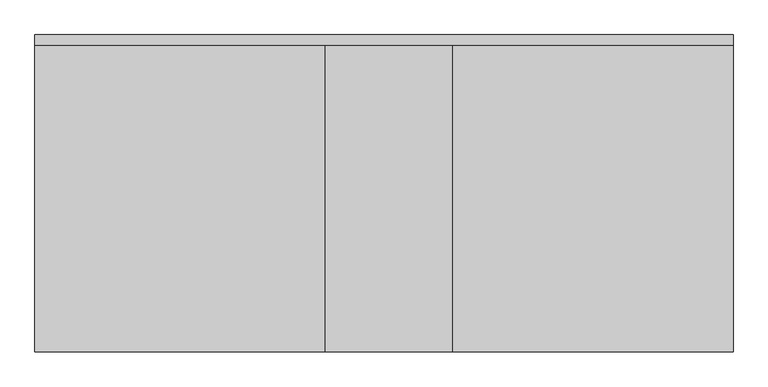
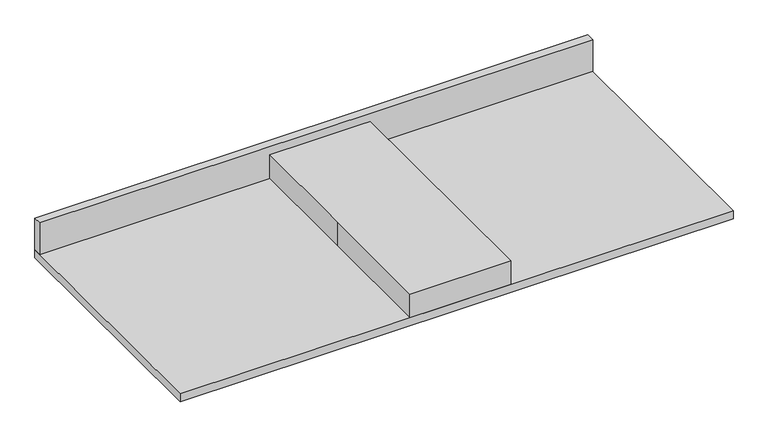
"""IFC4 building model written with IfcOpenShell, lengths in millimetres: proxy geometry, CT050 - Countertop, Stainless Steel (w-o opening) : CT050 - Countertop, Stainless Steel (w-o opening)."""

import ifcopenshell
import ifcopenshell.guid

model = None  # the IFC model being written
_history = None  # IfcOwnerHistory: only IFC2X3 demands one
_inside = {}  # id of a spatial element -> (the spatial element, [elements in it])
_under = {}  # id of a project, library or spatial element -> (it, [spatial elements below it])
_declared = {}  # id of a project -> (the project, [libraries it declares])
_typed = {}  # id of a type object -> (the type object, [elements of that type])
_made_of = {}  # id of a material, layer set ... -> (it, [elements and type objects made of it])


def new_model(schema):
    """Start an empty IFC model of exactly this schema.

    Asked for "IFC4X3", IfcOpenShell would pick the latest addendum, in which some entities
    have other attributes; the version numbers below select the first issue.
    IFC2X3 requires an IfcOwnerHistory on every rooted entity: one is made here for all.
    """
    global model, _history
    if schema == "IFC4X3":
        model = ifcopenshell.file(schema_version=(4, 3, 0, 0))
    else:
        model = ifcopenshell.file(schema=schema)
    _inside.clear()
    _under.clear()
    _declared.clear()
    _typed.clear()
    _made_of.clear()
    _history = None
    if model.schema == "IFC2X3":
        org = make("IfcOrganization", Name="unknown")
        user = make(
            "IfcPersonAndOrganization",
            ThePerson=make("IfcPerson", FamilyName="unknown"),
            TheOrganization=org,
        )
        app = make(
            "IfcApplication",
            ApplicationDeveloper=org,
            Version="unknown",
            ApplicationFullName="unknown",
            ApplicationIdentifier="unknown",
        )
        _history = make(
            "IfcOwnerHistory",
            OwningUser=user,
            OwningApplication=app,
            ChangeAction="ADDED",
            CreationDate=0,
        )
    return model


def make(cls, **values):
    """One entity of the class cls with the attributes given. An attribute that is None is left unset."""
    return model.create_entity(
        cls, **{name: value for name, value in values.items() if value is not None}
    )


def rooted(cls, **values):
    """An entity with a GlobalId (a new one), such as an element, a storey or a relation."""
    return make(cls, GlobalId=ifcopenshell.guid.new(), OwnerHistory=_history, **values)


def si_unit(unit_type, name, prefix=None):
    """IfcSIUnit, for example si_unit("LENGTHUNIT", "METRE", prefix="MILLI")."""
    return make("IfcSIUnit", UnitType=unit_type, Prefix=prefix, Name=name)


def assignment(units):
    """IfcUnitAssignment: the units of a project."""
    return None if units is None else make("IfcUnitAssignment", Units=units)


def point(xyz):
    """IfcCartesianPoint."""
    return None if xyz is None else make("IfcCartesianPoint", Coordinates=xyz)


def direction(xyz):
    """IfcDirection."""
    return None if xyz is None else make("IfcDirection", DirectionRatios=xyz)


def frame(location, z_axis=None, x_axis=None):
    """IfcAxis2Placement3D, a coordinate frame: its origin and axes. An axis left out is left unset."""
    return make(
        "IfcAxis2Placement3D",
        Location=point(location),
        Axis=direction(z_axis),
        RefDirection=direction(x_axis),
    )


def origin():
    """The frame at (0, 0, 0) with its axes left unset."""
    return frame((0.0, 0.0, 0.0))


def origin_with_axes():
    """The frame at (0, 0, 0) with the z axis (0, 0, 1) and the x axis (1, 0, 0) written out."""
    return frame((0.0, 0.0, 0.0), z_axis=(0.0, 0.0, 1.0), x_axis=(1.0, 0.0, 0.0))


def place(relative_to, where):
    """IfcLocalPlacement: puts the frame where relative to a parent placement (None: the world)."""
    return make(
        "IfcLocalPlacement", PlacementRelTo=relative_to, RelativePlacement=where
    )


def context(
    kind, dimensions, precision=None, world=None, true_north=None, identifier=None
):
    """IfcGeometricRepresentationContext, for example the 3D "Model" context."""
    return make(
        "IfcGeometricRepresentationContext",
        ContextIdentifier=identifier,
        ContextType=kind,
        CoordinateSpaceDimension=dimensions,
        Precision=precision,
        WorldCoordinateSystem=world,
        TrueNorth=true_north,
    )


def project(units=None, contexts=None):
    """IfcProject with its units and contexts."""
    return rooted(
        "IfcProject",
        Name="project",
        RepresentationContexts=contexts,
        UnitsInContext=assignment(units),
    )


def spatial(cls, under=None, at=None, **own):
    """A site, building, storey or space (cls), placed at a placement, below another one or the project."""
    s = rooted(cls, ObjectPlacement=at, **own)
    if under is not None:
        _under.setdefault(under.id(), (under, []))[1].append(s)
    return s


def polyline(points):
    """IfcPolyline through the points."""
    return make("IfcPolyline", Points=[point(p) for p in points])


def outline(outer, holes=None, kind="AREA"):
    """IfcArbitraryClosedProfileDef: a profile drawn as a closed curve; with holes, ...WithVoids."""
    if holes is None:
        return make("IfcArbitraryClosedProfileDef", ProfileType=kind, OuterCurve=outer)
    return make(
        "IfcArbitraryProfileDefWithVoids",
        ProfileType=kind,
        OuterCurve=outer,
        InnerCurves=holes,
    )


def extrude(swept, where, along, depth):
    """IfcExtrudedAreaSolid: the profile swept, set in the frame where, extruded along a direction by depth."""
    return make(
        "IfcExtrudedAreaSolid",
        SweptArea=swept,
        Position=where,
        ExtrudedDirection=direction(along),
        Depth=depth,
    )


def shape(context_of_items, identifier, shape_type, items):
    """IfcShapeRepresentation: the items that make up one representation, for example the "Body"."""
    return make(
        "IfcShapeRepresentation",
        ContextOfItems=context_of_items,
        RepresentationIdentifier=identifier,
        RepresentationType=shape_type,
        Items=items,
    )


def source(mapping_origin, context_of_items, identifier, shape_type, items):
    """IfcRepresentationMap: a shape defined once, which mapped items show again and again."""
    return make(
        "IfcRepresentationMap",
        MappingOrigin=mapping_origin,
        MappedRepresentation=shape(context_of_items, identifier, shape_type, items),
    )


def transform(
    local_origin,
    x_axis=None,
    y_axis=None,
    z_axis=None,
    scale=None,
    scale2=None,
    scale3=None,
    uniform=True,
):
    """IfcCartesianTransformationOperator3D, or its non-uniform kind. x_axis, y_axis, z_axis: its Axis1, 2, 3."""
    if uniform:
        return make(
            "IfcCartesianTransformationOperator3D",
            Axis1=direction(x_axis),
            Axis2=direction(y_axis),
            LocalOrigin=point(local_origin),
            Scale=scale,
            Axis3=direction(z_axis),
        )
    return make(
        "IfcCartesianTransformationOperator3DnonUniform",
        Axis1=direction(x_axis),
        Axis2=direction(y_axis),
        LocalOrigin=point(local_origin),
        Scale=scale,
        Axis3=direction(z_axis),
        Scale2=scale2,
        Scale3=scale3,
    )


def mapped(mapping_source, mapping_target):
    """IfcMappedItem: shows the shape of a source again, moved by a transform."""
    return make(
        "IfcMappedItem", MappingSource=mapping_source, MappingTarget=mapping_target
    )


def made_of(thing, what):
    """Note that an element or type object is made of a material, layer set ...; save() writes the relation."""
    if what is not None:
        _made_of.setdefault(what.id(), (what, []))[1].append(thing)
    return thing


def element(
    cls,
    number,
    at=None,
    inside=None,
    cuts=None,
    type_object=None,
    material=None,
    context=None,
    identifier="Body",
    shape_type=None,
    held_by="IfcProductDefinitionShape",
    body=None,
    shapes=None,
    **own,
):
    """One element of the class cls, such as IfcWall. Its Tag is "e" and its number.

    at: its placement. inside: the storey or other place that contains it. cuts: it is an
    opening in that element (IfcRelVoidsElement). A single representation is given by context,
    identifier, shape_type and body (its items); several are given by shapes. held_by: the class
    of the entity that holds the representations. save() writes the other relations.
    """
    e = rooted(cls, Tag="e%d" % number, ObjectPlacement=at, **own)
    if body is not None:
        shapes = [shape(context, identifier, shape_type, body)]
    if shapes is not None:
        e.Representation = make(held_by, Representations=shapes)
    if inside is not None:
        _inside.setdefault(inside.id(), (inside, []))[1].append(e)
    if cuts is not None:
        rooted(
            "IfcRelVoidsElement", RelatingBuildingElement=cuts, RelatedOpeningElement=e
        )
    if type_object is not None:
        _typed.setdefault(type_object.id(), (type_object, []))[1].append(e)
    return made_of(e, material)


def aggregate(whole, parts):
    """IfcRelAggregates: a whole, such as a stair, and the parts it consists of."""
    return rooted("IfcRelAggregates", RelatingObject=whole, RelatedObjects=parts)


def save(model, path):
    """Write the relations noted so far, then the file.

    IfcRelAggregates (storeys below a building ...), IfcRelContainedInSpatialStructure (elements
    in a storey), IfcRelDefinesByType, IfcRelAssociatesMaterial and IfcRelDeclares: one each for
    every whole, place, type object, material and project.
    """
    for whole, parts in _under.values():
        aggregate(whole, parts)
    for where, things in _inside.values():
        rooted(
            "IfcRelContainedInSpatialStructure",
            RelatedElements=things,
            RelatingStructure=where,
        )
    for kind, things in _typed.values():
        rooted("IfcRelDefinesByType", RelatedObjects=things, RelatingType=kind)
    for what, things in _made_of.values():
        rooted("IfcRelAssociatesMaterial", RelatedObjects=things, RelatingMaterial=what)
    for by, libraries in _declared.values():
        rooted("IfcRelDeclares", RelatingContext=by, RelatedDefinitions=libraries)
    model.write(path)


def specialty_equipment_aaaa1240(model_context):
    return source(origin(), model_context, "Body", "SweptSolid", [
        extrude(outline(polyline([(-849.3125, 355.6), (-849.3125, 381.0), (827.0875, 381.0), (827.0875, 355.6), (-849.3125, 355.6)])), frame((0.0, 0.0, 25.4), z_axis=(0.0, 0.0, 1.0), x_axis=(1.0, 0.0, 0.0)), (0.0, 0.0, 1.0), 101.6),
        extrude(outline(polyline([(827.0875, 381.0), (827.0875, -381.0), (-849.3125, -381.0), (-849.3125, 381.0), (827.0875, 381.0)])), origin_with_axes(), (0.0, 0.0, 1.0), 25.4),
        extrude(outline(polyline([(-152.4, 381.0), (152.4, 381.0), (152.4, -381.0), (-152.4, -381.0), (-152.4, 0.0), (-152.4, 381.0)])), origin_with_axes(), (0.0, 0.0, 1.0), 101.6),
    ])


if __name__ == "__main__":
    model = new_model("IFC4")
    model_context = context("Model", 3, world=origin())
    ifc_project = project(units=[si_unit("LENGTHUNIT", "METRE", prefix="MILLI")], contexts=[model_context])
    site = spatial("IfcSite", under=ifc_project)
    building = spatial("IfcBuilding", under=site)
    placement = place(None, origin())
    specialty_equipment_shape = specialty_equipment_aaaa1240(model_context)
    element("IfcBuildingElementProxy", 1, Name="CT050 - Countertop, Stainless Steel (w-o opening) : CT050 - Countertop, Stainless Steel (w-o opening)", ObjectType="CT050 - Countertop, Stainless Steel (w-o opening) : CT050 - Countertop, Stainless Steel (w-o opening)", at=placement, inside=building, context=model_context, shape_type="MappedRepresentation", body=[
        mapped(specialty_equipment_shape, transform((0.0, 0.0, 0.0), x_axis=(1.0, 0.0, 0.0), y_axis=(0.0, 1.0, 0.0), z_axis=(0.0, 0.0, 1.0))),
    ])
    save(model, "model.ifc")

# Revit data of these elements
# Project information
#   Room Abbreviation = "CSDE1"
#   Room Description = "Workroom, Sterile Processing, Decontamination (CSDE1)"
#   Sheets - Total = "7"
#   Project Issue Date = "Issue Date"
#   Project Status = "Project Status"
#   Client Name = "Owner"
#   Project Address = "Enter address here"
#   Project Name = "Project Name"
#   Project Number = "Project Number"
#   Publication Date = "30-Jan-15"
# Type "CT050 - Countertop, Stainless Steel (w-o opening) : CT050 - Countertop, Stainless Steel (w-o opening)"
#   Watts2 = "0"
#   Watts1 = "0"
#   Unit_Issue = "LF"
#   UTIL_6_Misc = "-"
#   UTIL_5_NonMedGas = "-"
#   UTIL_4_MiscGas = "-"
#   UTIL_3_MedGas = "-"
#   UTIL_2_Elec = "-"
#   UTIL_1_WaterDrain = "-"
#   Nomenclature = "Countertop, Stainless Steel"
#   NSN = "6530"
#   Location [instance default] = ""
#   JSN = "CT050"
#   Fund_Source_VA = "-"
#   Fund_Source_Navy = "-"
#   Fund_Source_Army = "-"
#   Fund_Source_AF = "-"
#   ELEC_Volts2 = "0"
#   ELEC_Volts1 = "0"
#   ELEC_Phase2 = "0"
#   ELEC_Phase1 = "0"
#   ELEC_HertzSwitch = "0"
#   ELEC_HertzDependent = "0"
#   ELEC_Hertz = "0"
#   ELEC_Amps2 = "0"
#   ELEC_Amps1 = "0"
#   DetailDescription = "Stainless steel countertop (composition of heavy-gauge Type No. 304 stainless steel) having a smooth satin finish and integral 4\" backsplash/curb. Also referred to as a corrosion-resistant steel work surface or work top. Available in various depths. Used in areas where excellent ease of cleaning, abrasion resistance, bacteria resistance, impact resistance, load capacity and moisture resistance, are of concern. Pricing based upon a 24\" depth."
#   CAT_VA = "A"
#   CAT_Navy = "A"
#   CAT_IHS = "-"
#   CAT_Army = "A"
#   CAT_AF = "A"
#   BTUperhour = "0"
#   Weight_IP = 0
#   OpeningLength [instance default] = 1' - 7"
#   OpeningDepth [instance default] = 1' - 4"
#   DIM_Width_IP = 1' - 0"
#   DIM_Height_IP = 0' - 4"
#   DIM_Depth_IP = 2' - 6"
#   CustomLength2 [instance default] = 1' - 6"
#   CustomLength [instance default] = 1' - 6"
#   Assembly Code = ""
# Element 1 (IfcBuildingElementProxy, "CT050 - Countertop, Stainless Steel (w-o opening) : CT050 - Countertop, Stainless Steel (w-o opening)")
#   Location = "CSDE2"
#   CustomLength2 = 2' - 8 9/16"
#   CustomLength = 2' - 9 7/16"
#   Materials on its faces: "CounterTopFinish - Stainless", "EquipSpace"
# Materials
#   "CounterTopFinish - Stainless": class "Unassigned", colour RGB 187 187 187, transparency 0
#   "EquipSpace": class "Unassigned", colour RGB 221 217 195, transparency 0.5
